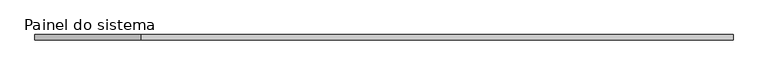
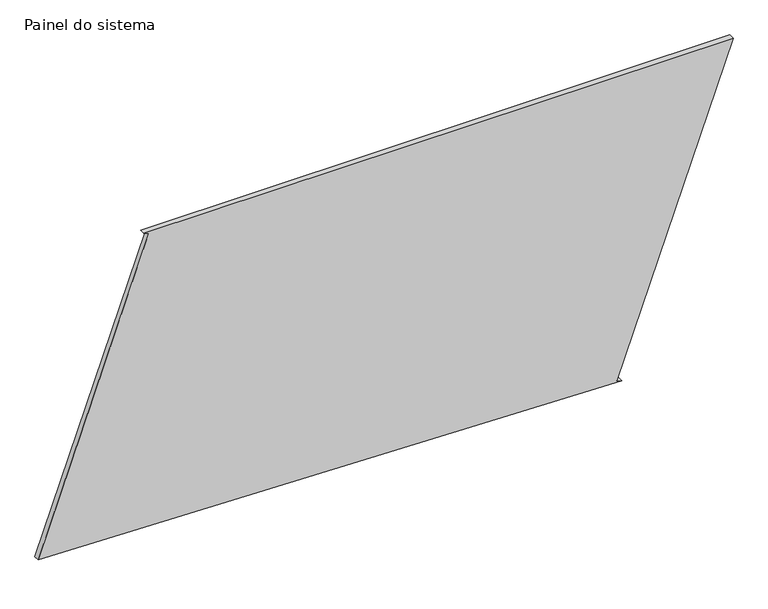
"""IFC4 building model written with IfcOpenShell, lengths in millimetres: plate geometry, Painel do sistema : Envidraçado."""

from ifc_helpers import new_model, si_unit, frame, origin, place, context, project, spatial, polyline, outline, extrude, source, transform, mapped, element, save


def painel_do_sistema_bcc91a5d(model_context):
    return source(origin(), model_context, "Body", "SweptSolid", [
        extrude(outline(polyline([(0.0, 1086.5182744), (8.505028, 1063.0094569), (1486.3515257, 1597.6652669), (1486.3515257, -1111.5617515), (1477.8464977, -1088.0529341), (69.22288, -1597.6652669), (0.0, 1086.5182744)])), frame((0.0, 24.5, 0.0), z_axis=(0.0, 1.0, 0.0), x_axis=(0.0, 0.0, 1.0)), (0.0, 0.0, 1.0), 25.0),
    ])


if __name__ == "__main__":
    model = new_model("IFC4")
    model_context = context("Model", 3, world=origin())
    ifc_project = project(units=[si_unit("LENGTHUNIT", "METRE", prefix="MILLI")], contexts=[model_context])
    site = spatial("IfcSite", under=ifc_project)
    building = spatial("IfcBuilding", under=site)
    placement = place(None, origin())
    painel_do_sistema_shape = painel_do_sistema_bcc91a5d(model_context)
    element("IfcPlate", 1, ObjectType="Painel do sistema : Envidraçado", at=placement, inside=building, context=model_context, shape_type="MappedRepresentation", body=[
        mapped(painel_do_sistema_shape, transform((0.0, 0.0, 0.0), x_axis=(1.0, 0.0, 0.0), y_axis=(0.0, 1.0, 0.0), z_axis=(0.0, 0.0, 1.0))),
    ])
    save(model, "model.ifc")

# Revit data of these elements
# Type "Painel do sistema : Envidraçado"
#   Construction Type Id = "GSP4R"
#   Analytic Construction = "Vidraça única Pilkington 1/8 pol"
#   Visual Light Transmittance = 0.9
#   Solar Heat Gain Coefficient = 0.86
#   Heat Transfer Coefficient (U) = 6.7069 W/(m²·K)
# Element 1 (IfcPlate, "Painel do sistema : Envidraçado")
#   Materials on its faces: "Vidro"
# Materials
#   "Vidro": class "Vidro", colour RGB 0 128 192, transparency 0.9, Description = "Vidro de sílica", Cost = 0
